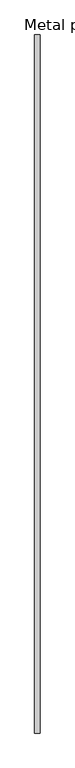
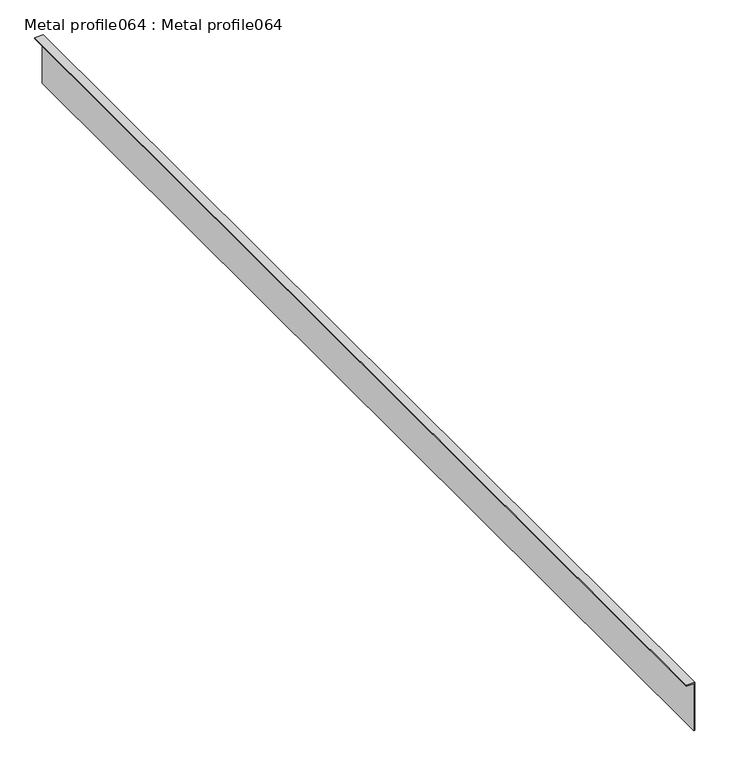
"""IFC4 building model written with IfcOpenShell, lengths in millimetres: proxy geometry, Metal profile064 : Metal profile064."""

import ifcopenshell
import ifcopenshell.guid

model = None  # the IFC model being written
_history = None  # IfcOwnerHistory: only IFC2X3 demands one
_inside = {}  # id of a spatial element -> (the spatial element, [elements in it])
_under = {}  # id of a project, library or spatial element -> (it, [spatial elements below it])
_declared = {}  # id of a project -> (the project, [libraries it declares])
_typed = {}  # id of a type object -> (the type object, [elements of that type])
_made_of = {}  # id of a material, layer set ... -> (it, [elements and type objects made of it])


def new_model(schema):
    """Start an empty IFC model of exactly this schema.

    Asked for "IFC4X3", IfcOpenShell would pick the latest addendum, in which some entities
    have other attributes; the version numbers below select the first issue.
    IFC2X3 requires an IfcOwnerHistory on every rooted entity: one is made here for all.
    """
    global model, _history
    if schema == "IFC4X3":
        model = ifcopenshell.file(schema_version=(4, 3, 0, 0))
    else:
        model = ifcopenshell.file(schema=schema)
    _inside.clear()
    _under.clear()
    _declared.clear()
    _typed.clear()
    _made_of.clear()
    _history = None
    if model.schema == "IFC2X3":
        org = make("IfcOrganization", Name="unknown")
        user = make(
            "IfcPersonAndOrganization",
            ThePerson=make("IfcPerson", FamilyName="unknown"),
            TheOrganization=org,
        )
        app = make(
            "IfcApplication",
            ApplicationDeveloper=org,
            Version="unknown",
            ApplicationFullName="unknown",
            ApplicationIdentifier="unknown",
        )
        _history = make(
            "IfcOwnerHistory",
            OwningUser=user,
            OwningApplication=app,
            ChangeAction="ADDED",
            CreationDate=0,
        )
    return model


def make(cls, **values):
    """One entity of the class cls with the attributes given. An attribute that is None is left unset."""
    return model.create_entity(
        cls, **{name: value for name, value in values.items() if value is not None}
    )


def rooted(cls, **values):
    """An entity with a GlobalId (a new one), such as an element, a storey or a relation."""
    return make(cls, GlobalId=ifcopenshell.guid.new(), OwnerHistory=_history, **values)


def si_unit(unit_type, name, prefix=None):
    """IfcSIUnit, for example si_unit("LENGTHUNIT", "METRE", prefix="MILLI")."""
    return make("IfcSIUnit", UnitType=unit_type, Prefix=prefix, Name=name)


def assignment(units):
    """IfcUnitAssignment: the units of a project."""
    return None if units is None else make("IfcUnitAssignment", Units=units)


def point(xyz):
    """IfcCartesianPoint."""
    return None if xyz is None else make("IfcCartesianPoint", Coordinates=xyz)


def direction(xyz):
    """IfcDirection."""
    return None if xyz is None else make("IfcDirection", DirectionRatios=xyz)


def frame(location, z_axis=None, x_axis=None):
    """IfcAxis2Placement3D, a coordinate frame: its origin and axes. An axis left out is left unset."""
    return make(
        "IfcAxis2Placement3D",
        Location=point(location),
        Axis=direction(z_axis),
        RefDirection=direction(x_axis),
    )


def origin():
    """The frame at (0, 0, 0) with its axes left unset."""
    return frame((0.0, 0.0, 0.0))


def place(relative_to, where):
    """IfcLocalPlacement: puts the frame where relative to a parent placement (None: the world)."""
    return make(
        "IfcLocalPlacement", PlacementRelTo=relative_to, RelativePlacement=where
    )


def context(
    kind, dimensions, precision=None, world=None, true_north=None, identifier=None
):
    """IfcGeometricRepresentationContext, for example the 3D "Model" context."""
    return make(
        "IfcGeometricRepresentationContext",
        ContextIdentifier=identifier,
        ContextType=kind,
        CoordinateSpaceDimension=dimensions,
        Precision=precision,
        WorldCoordinateSystem=world,
        TrueNorth=true_north,
    )


def project(units=None, contexts=None):
    """IfcProject with its units and contexts."""
    return rooted(
        "IfcProject",
        Name="project",
        RepresentationContexts=contexts,
        UnitsInContext=assignment(units),
    )


def spatial(cls, under=None, at=None, **own):
    """A site, building, storey or space (cls), placed at a placement, below another one or the project."""
    s = rooted(cls, ObjectPlacement=at, **own)
    if under is not None:
        _under.setdefault(under.id(), (under, []))[1].append(s)
    return s


def polyline(points):
    """IfcPolyline through the points."""
    return make("IfcPolyline", Points=[point(p) for p in points])


def outline(outer, holes=None, kind="AREA"):
    """IfcArbitraryClosedProfileDef: a profile drawn as a closed curve; with holes, ...WithVoids."""
    if holes is None:
        return make("IfcArbitraryClosedProfileDef", ProfileType=kind, OuterCurve=outer)
    return make(
        "IfcArbitraryProfileDefWithVoids",
        ProfileType=kind,
        OuterCurve=outer,
        InnerCurves=holes,
    )


def extrude(swept, where, along, depth):
    """IfcExtrudedAreaSolid: the profile swept, set in the frame where, extruded along a direction by depth."""
    return make(
        "IfcExtrudedAreaSolid",
        SweptArea=swept,
        Position=where,
        ExtrudedDirection=direction(along),
        Depth=depth,
    )


def shape(context_of_items, identifier, shape_type, items):
    """IfcShapeRepresentation: the items that make up one representation, for example the "Body"."""
    return make(
        "IfcShapeRepresentation",
        ContextOfItems=context_of_items,
        RepresentationIdentifier=identifier,
        RepresentationType=shape_type,
        Items=items,
    )


def source(mapping_origin, context_of_items, identifier, shape_type, items):
    """IfcRepresentationMap: a shape defined once, which mapped items show again and again."""
    return make(
        "IfcRepresentationMap",
        MappingOrigin=mapping_origin,
        MappedRepresentation=shape(context_of_items, identifier, shape_type, items),
    )


def transform(
    local_origin,
    x_axis=None,
    y_axis=None,
    z_axis=None,
    scale=None,
    scale2=None,
    scale3=None,
    uniform=True,
):
    """IfcCartesianTransformationOperator3D, or its non-uniform kind. x_axis, y_axis, z_axis: its Axis1, 2, 3."""
    if uniform:
        return make(
            "IfcCartesianTransformationOperator3D",
            Axis1=direction(x_axis),
            Axis2=direction(y_axis),
            LocalOrigin=point(local_origin),
            Scale=scale,
            Axis3=direction(z_axis),
        )
    return make(
        "IfcCartesianTransformationOperator3DnonUniform",
        Axis1=direction(x_axis),
        Axis2=direction(y_axis),
        LocalOrigin=point(local_origin),
        Scale=scale,
        Axis3=direction(z_axis),
        Scale2=scale2,
        Scale3=scale3,
    )


def mapped(mapping_source, mapping_target):
    """IfcMappedItem: shows the shape of a source again, moved by a transform."""
    return make(
        "IfcMappedItem", MappingSource=mapping_source, MappingTarget=mapping_target
    )


def made_of(thing, what):
    """Note that an element or type object is made of a material, layer set ...; save() writes the relation."""
    if what is not None:
        _made_of.setdefault(what.id(), (what, []))[1].append(thing)
    return thing


def element(
    cls,
    number,
    at=None,
    inside=None,
    cuts=None,
    type_object=None,
    material=None,
    context=None,
    identifier="Body",
    shape_type=None,
    held_by="IfcProductDefinitionShape",
    body=None,
    shapes=None,
    **own,
):
    """One element of the class cls, such as IfcWall. Its Tag is "e" and its number.

    at: its placement. inside: the storey or other place that contains it. cuts: it is an
    opening in that element (IfcRelVoidsElement). A single representation is given by context,
    identifier, shape_type and body (its items); several are given by shapes. held_by: the class
    of the entity that holds the representations. save() writes the other relations.
    """
    e = rooted(cls, Tag="e%d" % number, ObjectPlacement=at, **own)
    if body is not None:
        shapes = [shape(context, identifier, shape_type, body)]
    if shapes is not None:
        e.Representation = make(held_by, Representations=shapes)
    if inside is not None:
        _inside.setdefault(inside.id(), (inside, []))[1].append(e)
    if cuts is not None:
        rooted(
            "IfcRelVoidsElement", RelatingBuildingElement=cuts, RelatedOpeningElement=e
        )
    if type_object is not None:
        _typed.setdefault(type_object.id(), (type_object, []))[1].append(e)
    return made_of(e, material)


def aggregate(whole, parts):
    """IfcRelAggregates: a whole, such as a stair, and the parts it consists of."""
    return rooted("IfcRelAggregates", RelatingObject=whole, RelatedObjects=parts)


def save(model, path):
    """Write the relations noted so far, then the file.

    IfcRelAggregates (storeys below a building ...), IfcRelContainedInSpatialStructure (elements
    in a storey), IfcRelDefinesByType, IfcRelAssociatesMaterial and IfcRelDeclares: one each for
    every whole, place, type object, material and project.
    """
    for whole, parts in _under.values():
        aggregate(whole, parts)
    for where, things in _inside.values():
        rooted(
            "IfcRelContainedInSpatialStructure",
            RelatedElements=things,
            RelatingStructure=where,
        )
    for kind, things in _typed.values():
        rooted("IfcRelDefinesByType", RelatedObjects=things, RelatingType=kind)
    for what, things in _made_of.values():
        rooted("IfcRelAssociatesMaterial", RelatedObjects=things, RelatingMaterial=what)
    for by, libraries in _declared.values():
        rooted("IfcRelDeclares", RelatingContext=by, RelatedDefinitions=libraries)
    model.write(path)


def metal_profile064_metal_profile064_f35a4d71(model_context):
    return source(origin(), model_context, "Body", "SweptSolid", [
        extrude(outline(polyline([(42129.6796875, -1107.2874756), (42129.6796875, -1094.2821045), (42042.0195312, -1094.2821045), (42042.0195312, -1092.2821045), (42131.6796875, -1092.2821045), (42131.6796875, -1107.2874756), (42129.6796875, -1107.2874756)])), frame((0.0, -1052.8906574, 0.0), z_axis=(0.0, 1.0, 0.0), x_axis=(0.0, 0.0, 1.0)), (0.0, 0.0, 1.0), 2000.0),
    ])


if __name__ == "__main__":
    model = new_model("IFC4")
    model_context = context("Model", 3, world=origin())
    ifc_project = project(units=[si_unit("LENGTHUNIT", "METRE", prefix="MILLI")], contexts=[model_context])
    site = spatial("IfcSite", under=ifc_project)
    building = spatial("IfcBuilding", under=site)
    placement = place(None, origin())
    metal_profile064_metal_profile064_shape = metal_profile064_metal_profile064_f35a4d71(model_context)
    element("IfcBuildingElementProxy", 1, Name="Metal profile064 : Metal profile064", ObjectType="Metal profile064 : Metal profile064", at=placement, inside=building, context=model_context, shape_type="MappedRepresentation", body=[
        mapped(metal_profile064_metal_profile064_shape, transform((0.0, 0.0, 0.0), x_axis=(1.0, 0.0, 0.0), y_axis=(0.0, 1.0, 0.0), z_axis=(0.0, 0.0, 1.0))),
    ])
    save(model, "model.ifc")

# Revit data of these elements
# Type "Metal profile064 : Metal profile064"
#   NameOverride = "Metal profile064"
# Element 1 (IfcBuildingElementProxy, "Metal profile064 : Metal profile064")
#   Materials on its faces: "L-SHAPED METAL TRIM"
# Materials
#   "L-SHAPED METAL TRIM": class "Unassigned", colour RGB 255 231 0, transparency 0
